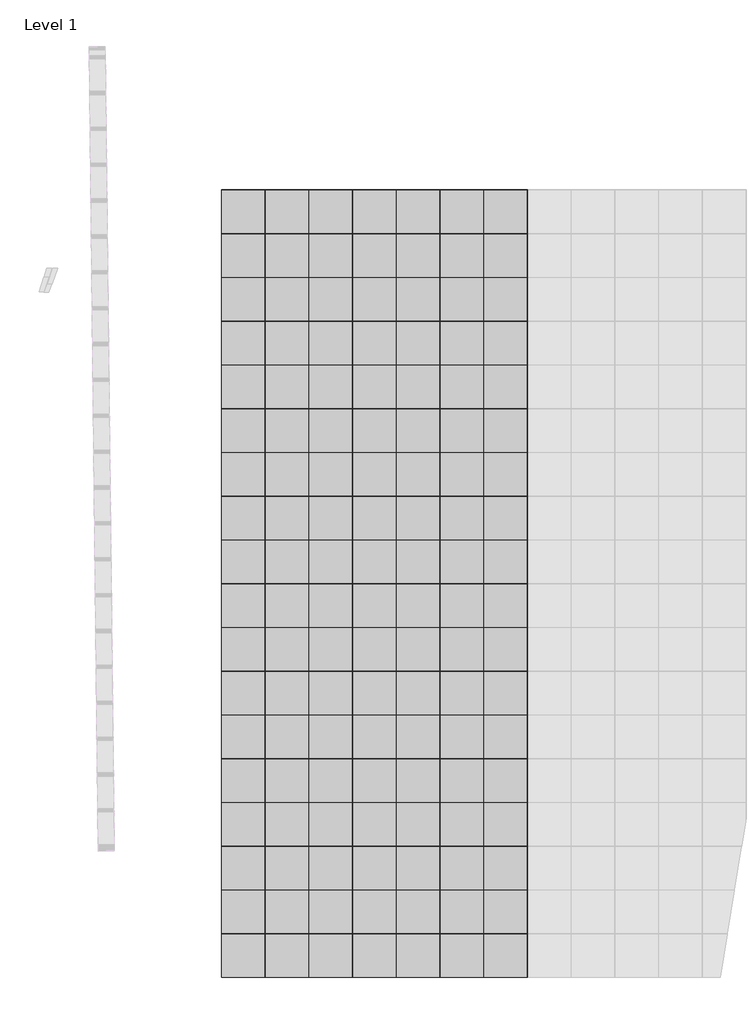
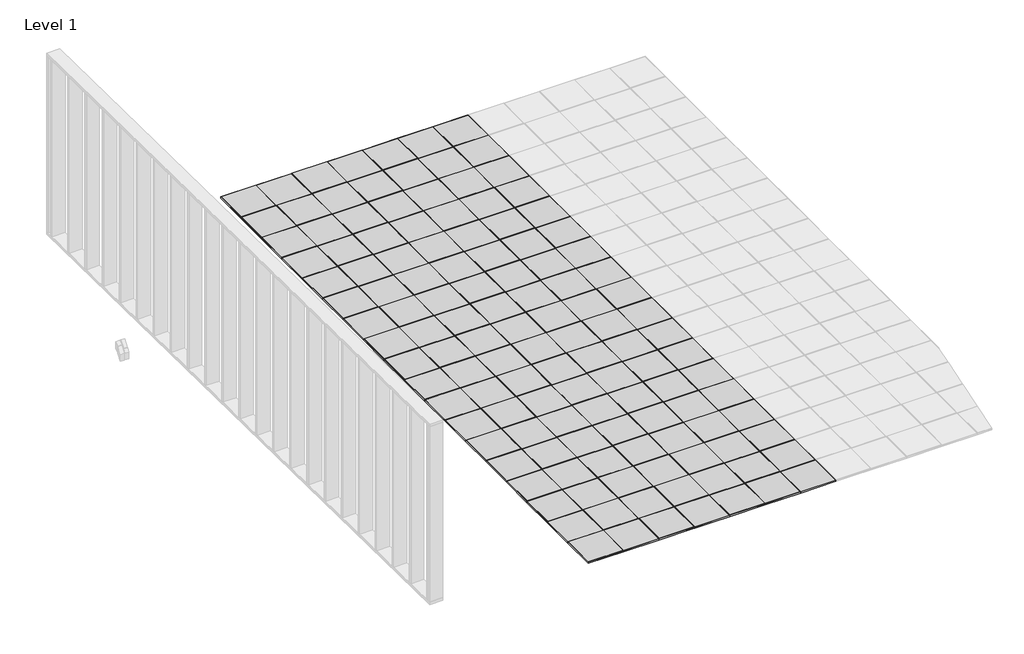
# One storey, part 1 of 18: 126 plates.
# Revit data of these elements (continued)
# Materials (continued)
#   "20_voeg": class "Concrete", colour RGB 86 86 86, transparency 0, Manufacturer = "RevitGG", URL = "www.revitgg.nl", Description = "zandcement, generiek materiaal", Cost = 0
#   "300_hardsteen_zwart": class "Generic", colour RGB 15 15 15, transparency 0, Description = "kalkzandsteen", Cost = 0
